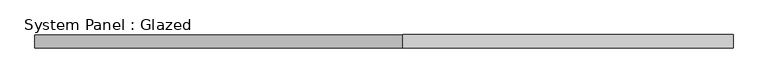
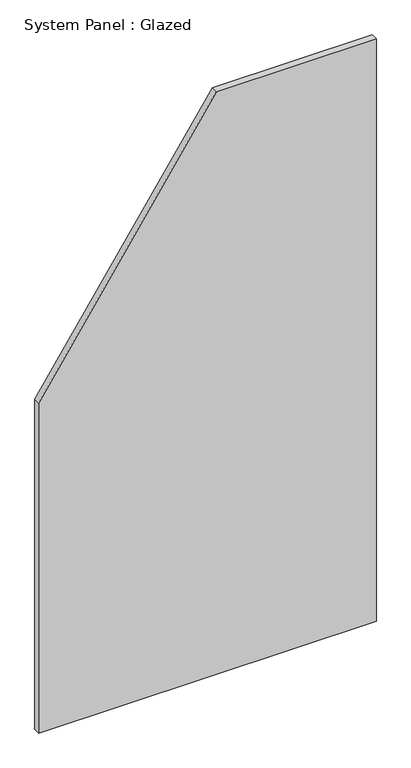
"""IFC4 building model written with IfcOpenShell, lengths in millimetres: plate geometry, System Panel : Glazed."""

from ifc_helpers import new_model, si_unit, frame, origin, place, context, project, spatial, polyline, outline, extrude, source, transform, mapped, element, save


def system_panel_glazed_919a12bb(model_context):
    return source(origin(), model_context, "Body", "SweptSolid", [
        extrude(outline(polyline([(0.0, -658.3333333), (0.0, 658.3333333), (2400.0, 658.3333333), (2400.0, 35.3849432), (1359.5656239, -658.3333333), (0.0, -658.3333333)])), frame((0.0, 24.5, 0.0), z_axis=(0.0, 1.0, 0.0), x_axis=(0.0, 0.0, 1.0)), (0.0, 0.0, 1.0), 25.0),
    ])


if __name__ == "__main__":
    model = new_model("IFC4")
    model_context = context("Model", 3, world=origin())
    ifc_project = project(units=[si_unit("LENGTHUNIT", "METRE", prefix="MILLI")], contexts=[model_context])
    site = spatial("IfcSite", under=ifc_project)
    building = spatial("IfcBuilding", under=site)
    placement = place(None, origin())
    system_panel_glazed_shape = system_panel_glazed_919a12bb(model_context)
    element("IfcPlate", 1, ObjectType="System Panel : Glazed", at=placement, inside=building, context=model_context, shape_type="MappedRepresentation", body=[
        mapped(system_panel_glazed_shape, transform((0.0, 0.0, 0.0), x_axis=(1.0, 0.0, 0.0), y_axis=(0.0, 1.0, 0.0), z_axis=(0.0, 0.0, 1.0))),
    ])
    save(model, "model.ifc")

# Revit data of these elements
# Type "System Panel : Glazed"
#   Keynote = "H11"
#   Construction Type Id = "GSP4R"
#   Analytic Construction = "1/8 in Pilkington single glazing"
#   Visual Light Transmittance = 0.9
#   Solar Heat Gain Coefficient = 0.86
#   Heat Transfer Coefficient (U) = 6.7069 W/(m²·K)
#   Define Thermal Properties by = 1
# Element 1 (IfcPlate, "System Panel : Glazed")
#   Materials on its faces: "Glass"
# Materials
#   "Glass": class "Glass", colour RGB 0 128 192, transparency 0.9, Description = "Soda Lime Glass", Cost = 0
